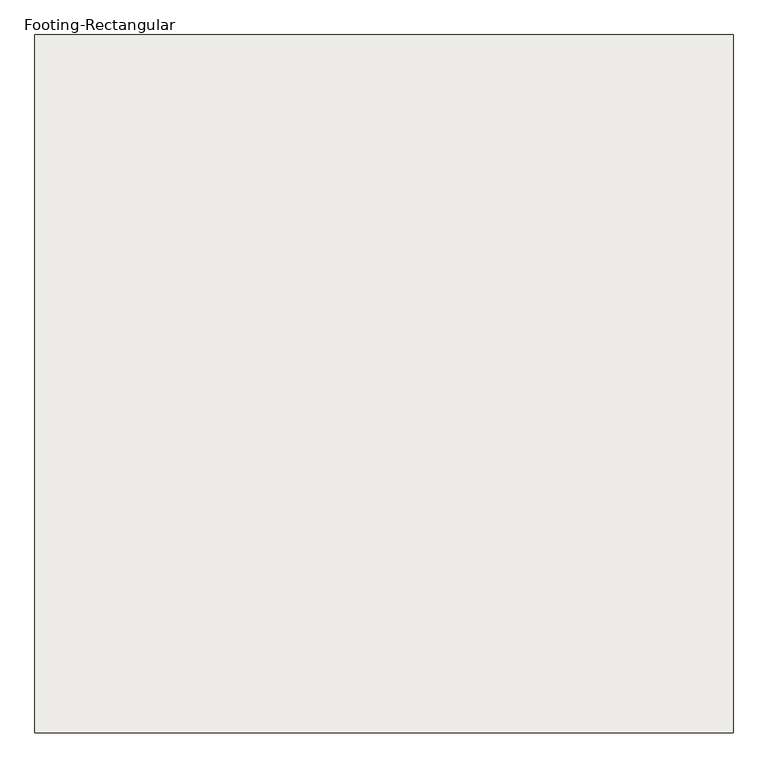
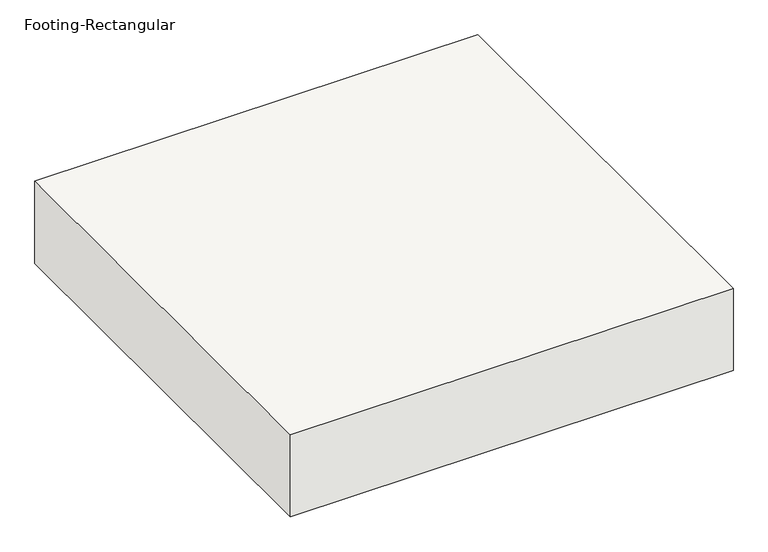
"""IFC4 building model written with IfcOpenShell, lengths in millimetres: slab geometry, Footing-Rectangular."""

from ifc_helpers import new_model, si_unit, frame, origin, place, context, project, spatial, polyline, outline, extrude, source, transform, mapped, element, save


def footing_rectangular_0e916acc(model_context):
    return source(origin(), model_context, "Body", "SweptSolid", [
        extrude(outline(polyline([(1295.4, 1295.4), (1295.4, -1295.4), (-1295.4, -1295.4), (-1295.4, 1295.4), (1295.4, 1295.4)])), frame((0.0, 0.0, -508.0), z_axis=(0.0, 0.0, 1.0), x_axis=(1.0, 0.0, 0.0)), (0.0, 0.0, 1.0), 508.0),
    ])


if __name__ == "__main__":
    model = new_model("IFC4")
    model_context = context("Model", 3, world=origin())
    ifc_project = project(units=[si_unit("LENGTHUNIT", "METRE", prefix="MILLI")], contexts=[model_context])
    site = spatial("IfcSite", under=ifc_project)
    building = spatial("IfcBuilding", under=site)
    placement = place(None, origin())
    footing_rectangular_shape = footing_rectangular_0e916acc(model_context)
    element("IfcSlab", 1, ObjectType="Footing-Rectangular : H 8.5' x 8.5' x 20\"", at=placement, inside=building, context=model_context, shape_type="MappedRepresentation", body=[
        mapped(footing_rectangular_shape, transform((0.0, 0.0, 0.0), x_axis=(1.0, 0.0, 0.0), y_axis=(0.0, 1.0, 0.0), z_axis=(0.0, 0.0, 1.0))),
    ])
    save(model, "model.ifc")

# Revit data of these elements
# Type "Footing-Rectangular : H 8.5' x 8.5' x 20\""
#   Assembly Code = "A1010100"
#   Width = 8' - 6"
#   Length = 8' - 6"
#   Foundation Thickness = 1' - 8"
#   Structural Material [instance default] = Concrete, Cast-in-Place gray
# Element 1 (IfcSlab, "Footing-Rectangular : H 8.5' x 8.5' x 20\"")
#   Materials on its faces: "Concrete, Cast-in-Place gray"
# Materials
#   "Concrete, Cast-in-Place gray": class "Concrete", colour RGB 192 192 192, transparency 0, Description = "Cast-in-place concrete", Cost = 0
